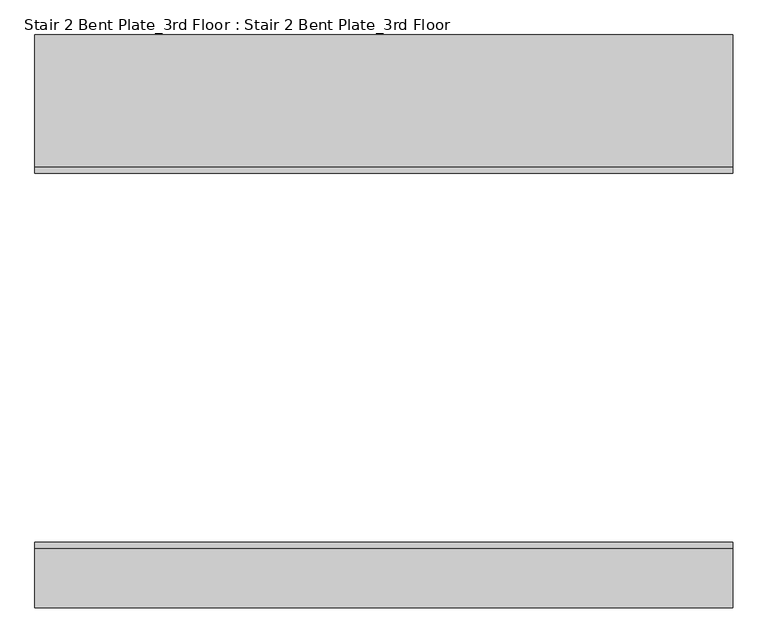
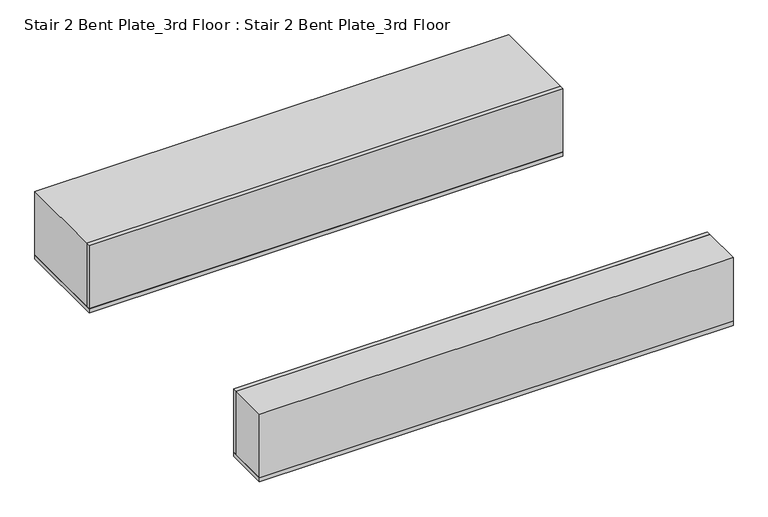
"""IFC4 building model written with IfcOpenShell, lengths in millimetres: proxy geometry, Stair 2 Bent Plate_3rd Floor : Stair 2 Bent Plate_3rd Floor."""

from ifc_helpers import new_model, si_unit, frame, origin, origin_with_axes, place, context, project, spatial, polyline, outline, extrude, source, transform, mapped, element, save


def stair_2_bent_plate_3rd_floor_stair_2_bent_plate_3rd_floor_afa8fdab(model_context):
    return source(origin(), model_context, "Body", "SweptSolid", [
        extrude(outline(polyline([(-247.65, -828.675), (-247.65, -714.375), (1098.55, -714.375), (1098.55, -828.675), (-247.65, -828.675)])), frame((0.0, 0.0, 12.7), z_axis=(0.0, 0.0, 1.0), x_axis=(1.0, 0.0, 0.0)), (0.0, 0.0, 1.0), 190.5),
        extrude(outline(polyline([(1098.55, 276.225), (1098.55, 22.225), (-247.65, 22.225), (-247.65, 276.225), (1098.55, 276.225)])), frame((0.0, 0.0, 12.7), z_axis=(0.0, 0.0, 1.0), x_axis=(1.0, 0.0, 0.0)), (0.0, 0.0, 1.0), 190.5),
        extrude(outline(polyline([(1098.55, -828.675), (-247.65, -828.675), (-247.65, -701.675), (1098.55, -701.675), (1098.55, -828.675)])), origin_with_axes(), (0.0, 0.0, 1.0), 12.7),
        extrude(outline(polyline([(1098.55, 9.525), (-247.65, 9.525), (-247.65, 276.225), (1098.55, 276.225), (1098.55, 9.525)])), origin_with_axes(), (0.0, 0.0, 1.0), 12.7),
        extrude(outline(polyline([(-247.65, -701.675), (1098.55, -701.675), (1098.55, -714.375), (-247.65, -714.375), (-247.65, -701.675)])), origin_with_axes(), (0.0, 0.0, 1.0), 203.2),
        extrude(outline(polyline([(1098.55, 9.525), (-247.65, 9.525), (-247.65, 22.225), (1098.55, 22.225), (1098.55, 9.525)])), origin_with_axes(), (0.0, 0.0, 1.0), 203.2),
    ])


if __name__ == "__main__":
    model = new_model("IFC4")
    model_context = context("Model", 3, world=origin())
    ifc_project = project(units=[si_unit("LENGTHUNIT", "METRE", prefix="MILLI")], contexts=[model_context])
    site = spatial("IfcSite", under=ifc_project)
    building = spatial("IfcBuilding", under=site)
    placement = place(None, origin())
    stair_2_bent_plate_3rd_floor_stair_2_bent_plate_3rd_floor_shape = stair_2_bent_plate_3rd_floor_stair_2_bent_plate_3rd_floor_afa8fdab(model_context)
    element("IfcBuildingElementProxy", 1, Name="Stair 2 Bent Plate_3rd Floor : Stair 2 Bent Plate_3rd Floor", ObjectType="Stair 2 Bent Plate_3rd Floor : Stair 2 Bent Plate_3rd Floor", at=placement, inside=building, context=model_context, shape_type="MappedRepresentation", body=[
        mapped(stair_2_bent_plate_3rd_floor_stair_2_bent_plate_3rd_floor_shape, transform((0.0, 0.0, 0.0), x_axis=(1.0, 0.0, 0.0), y_axis=(0.0, 1.0, 0.0), z_axis=(0.0, 0.0, 1.0))),
    ])
    save(model, "model.ifc")

# Revit data of these elements
# Element 1 (IfcBuildingElementProxy, "Stair 2 Bent Plate_3rd Floor : Stair 2 Bent Plate_3rd Floor")
#   Materials on its faces: "Concrete Infill"
# Materials
#   "Concrete Infill": class "Generic", colour RGB 0 255 0, transparency 0, Cost = 0
